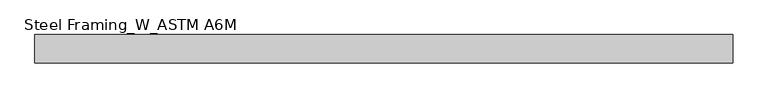
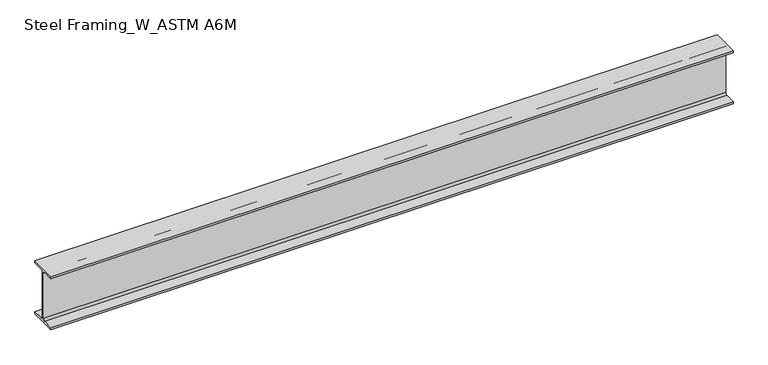
"""IFC4 building model written with IfcOpenShell, lengths in millimetres: beam geometry, Steel Framing_W_ASTM A6M : H_SB_AR_S02_W200x22.5_J1."""

from ifc_helpers import new_model, si_unit, point, frame, frame_2d, origin, place, context, project, spatial, polyline, circle_curve, trimmed, segment, composite_curve, outline, extrude, source, transform, mapped, element, save


def steel_framing_w_astm_a6m_abf0dccc(model_context):
    return source(origin(), model_context, "Body", "SweptSolid", [
        extrude(outline(composite_curve([segment(polyline([(51.0, -95.0), (51.0, -103.0), (-51.0, -103.0), (-51.0, -95.0), (-10.71, -95.0)]), True, "CONTINUOUS"), segment(trimmed(circle_curve(frame_2d((-10.71, -87.4)), 7.6), [point((-10.71, -95.0))], [point((-3.11, -87.4))], True, "CARTESIAN"), True, "CONTINUOUS"), segment(polyline([(-3.11, -87.4), (-3.11, 87.4)]), True, "CONTINUOUS"), segment(trimmed(circle_curve(frame_2d((-10.71, 87.4)), 7.6), [point((-3.11, 87.4))], [point((-10.71, 95.0))], True, "CARTESIAN"), True, "CONTINUOUS"), segment(polyline([(-10.71, 95.0), (-51.0, 95.0), (-51.0, 103.0), (51.0, 103.0), (51.0, 95.0), (10.71, 95.0)]), True, "CONTINUOUS"), segment(trimmed(circle_curve(frame_2d((10.71, 87.4)), 7.6), [point((10.71, 95.0))], [point((3.11, 87.4))], True, "CARTESIAN"), True, "CONTINUOUS"), segment(polyline([(3.11, 87.4), (3.11, -87.4)]), True, "CONTINUOUS"), segment(trimmed(circle_curve(frame_2d((10.71, -87.4)), 7.6), [point((3.11, -87.4))], [point((10.71, -95.0))], True, "CARTESIAN"), True, "CONTINUOUS"), segment(polyline([(10.71, -95.0), (51.0, -95.0)]), True, "CONTINUOUS")], self_intersect=False)), frame((-1319.7, 0.0, 0.0), z_axis=(1.0, 0.0, 0.0), x_axis=(0.0, 1.0, 0.0)), (0.0, 0.0, 1.0), 2512.5),
    ])


if __name__ == "__main__":
    model = new_model("IFC4")
    model_context = context("Model", 3, world=origin())
    ifc_project = project(units=[si_unit("LENGTHUNIT", "METRE", prefix="MILLI")], contexts=[model_context])
    site = spatial("IfcSite", under=ifc_project)
    building = spatial("IfcBuilding", under=site)
    placement = place(None, origin())
    steel_framing_w_astm_a6m_shape = steel_framing_w_astm_a6m_abf0dccc(model_context)
    element("IfcBeam", 1, ObjectType="Steel Framing_W_ASTM A6M : H_SB_AR_S02_W200x22.5_J1", at=placement, inside=building, context=model_context, shape_type="MappedRepresentation", body=[
        mapped(steel_framing_w_astm_a6m_shape, transform((0.0, 0.0, 0.0), x_axis=(1.0, 0.0, 0.0), y_axis=(0.0, 1.0, 0.0), z_axis=(0.0, 0.0, 1.0))),
    ])
    save(model, "model.ifc")

# Revit data of these elements
# Type "Steel Framing_W_ASTM A6M : H_SB_AR_S02_W200x22.5_J1"
#   Section Name Key = "W8x15"
#   Width = 10.2 cm
#   Web Thickness = 0.622 cm
#   Web Fillet = 0.76 cm
#   Warping Constant = 13900.0 cm⁶
#   Torsional Moment of Inertia = 5.70 cm⁴
#   Section Area = 28.6 cm²
#   Plastic Modulus weak axis = 43.8 cm³
#   Plastic Modulus strong axis = 223.0 cm³
#   Perimeter = 0.795 m²/m
#   Nominal Weight = 22.50 kgf/m
#   Moment of Inertia weak axis = 142.00 cm⁴
#   Moment of Inertia strong axis = 2000.00 cm⁴
#   Height = 20.6 cm
#   Flange Thickness = 0.8 cm
#   Elastic Modulus weak axis = 27.9 cm³
#   Elastic Modulus strong axis = 193.0 cm³
#   Centroid Vertical = 10.3 cm
#   Centroid Horizontal = 5.1 cm
#   Length [instance default] = 1500 mm
#   Structural Material [instance default] = Steel, 45-345
#   Bolt Spacing = 0
#   Assembly Code = ""
# Element 1 (IfcBeam, "Steel Framing_W_ASTM A6M : H_SB_AR_S02_W200x22.5_J1")
#   Materials on its faces: "Steel, 45-345"
# Materials
#   "Steel, 45-345": class "Metal", colour RGB 189 187 185, transparency 0, Description = "Steel 345 MPa", Cost = 0
